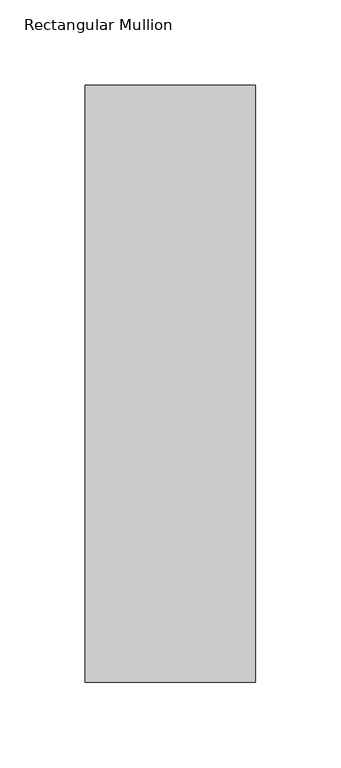
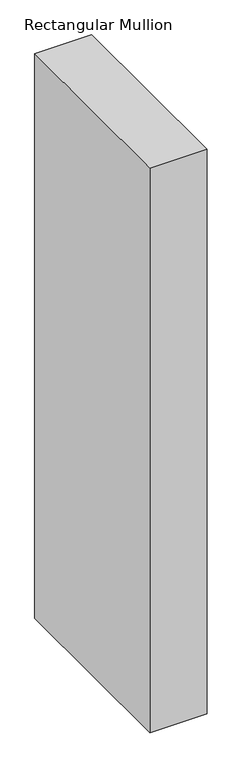
"""IFC4 building model written with IfcOpenShell, lengths in millimetres: member geometry, Rectangular Mullion : WWm-100x350-100mmOffset."""

from ifc_helpers import new_model, si_unit, frame, origin, place, context, project, spatial, polyline, outline, extrude, source, transform, mapped, element, save


def rectangular_mullion_28895888(model_context):
    return source(origin(), model_context, "Body", "SweptSolid", [
        extrude(outline(polyline([(0.0, 175.0), (0.0, -175.0), (-100.0, -175.0), (-100.0, 175.0), (0.0, 175.0)])), frame((0.0, 0.0, -1046.8563766), z_axis=(0.0, 0.0, 1.0), x_axis=(1.0, 0.0, 0.0)), (0.0, 0.0, 1.0), 1046.8563766),
    ])


if __name__ == "__main__":
    model = new_model("IFC4")
    model_context = context("Model", 3, world=origin())
    ifc_project = project(units=[si_unit("LENGTHUNIT", "METRE", prefix="MILLI")], contexts=[model_context])
    site = spatial("IfcSite", under=ifc_project)
    building = spatial("IfcBuilding", under=site)
    placement = place(None, origin())
    rectangular_mullion_shape = rectangular_mullion_28895888(model_context)
    element("IfcMember", 1, ObjectType="Rectangular Mullion : WWm-100x350-100mmOffset", at=placement, inside=building, context=model_context, shape_type="MappedRepresentation", body=[
        mapped(rectangular_mullion_shape, transform((0.0, 0.0, 0.0), x_axis=(1.0, 0.0, 0.0), y_axis=(0.0, 1.0, 0.0), z_axis=(0.0, 0.0, 1.0))),
    ])
    save(model, "model.ifc")

# Revit data of these elements
# Type "Rectangular Mullion : WWm-100x350-100mmOffset"
#   built-in parameter 1007304 = 1.14829 (stored number, unit not read)
#   built-in parameter 1007301 = 0.164042 (stored number, unit not read)
#   built-in parameter 1007300 = 0.164042 (stored number, unit not read)
# Element 1 (IfcMember, "Rectangular Mullion : WWm-100x350-100mmOffset")
#   Materials on its faces: "WW-EC-RGB-Mullion"
# Materials
#   "WW-EC-RGB-Mullion": class "Generic", colour RGB 255 255 255, transparency 0, Comments = "If region requests black mullions, switch asset color to RGB 25-25-25", Description = "Generic Color", Cost = 0
